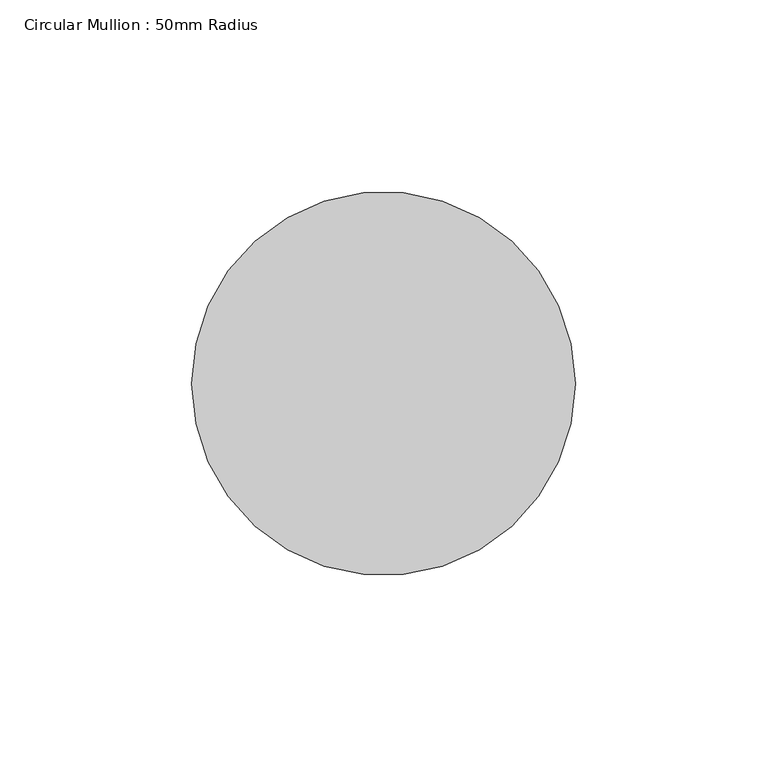
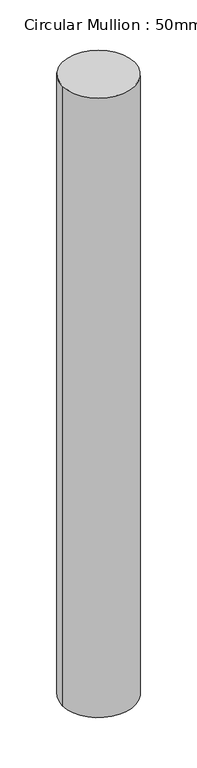
"""IFC4 building model written with IfcOpenShell, lengths in millimetres: member geometry, Circular Mullion : 50mm Radius."""

from ifc_helpers import new_model, si_unit, point, frame, origin, origin_2d, place, context, project, spatial, circle_curve, trimmed, segment, composite_curve, outline, extrude, source, transform, mapped, element, save


def circular_mullion_50mm_radius_d6f7776c(model_context):
    return source(origin(), model_context, "Body", "SweptSolid", [
        extrude(outline(composite_curve([segment(trimmed(circle_curve(origin_2d(), 50.0), [point((50.0, 0.0))], [point((-50.0, 0.0))], False, "CARTESIAN"), True, "CONTINUOUS"), segment(trimmed(circle_curve(origin_2d(), 50.0), [point((-50.0, 0.0))], [point((50.0, 0.0))], False, "CARTESIAN"), True, "CONTINUOUS")], self_intersect=False)), frame((0.0, 0.0, -908.470151), z_axis=(0.0, 0.0, 1.0), x_axis=(1.0, 0.0, 0.0)), (0.0, 0.0, 1.0), 908.470151),
    ])


if __name__ == "__main__":
    model = new_model("IFC4")
    model_context = context("Model", 3, world=origin())
    ifc_project = project(units=[si_unit("LENGTHUNIT", "METRE", prefix="MILLI")], contexts=[model_context])
    site = spatial("IfcSite", under=ifc_project)
    building = spatial("IfcBuilding", under=site)
    placement = place(None, origin())
    circular_mullion_50mm_radius_shape = circular_mullion_50mm_radius_d6f7776c(model_context)
    element("IfcMember", 1, ObjectType="Circular Mullion : 50mm Radius", at=placement, inside=building, context=model_context, shape_type="MappedRepresentation", body=[
        mapped(circular_mullion_50mm_radius_shape, transform((0.0, 0.0, 0.0), x_axis=(1.0, 0.0, 0.0), y_axis=(0.0, 1.0, 0.0), z_axis=(0.0, 0.0, 1.0))),
    ])
    save(model, "model.ifc")

# Revit data of these elements
# Type "Circular Mullion : 50mm Radius"
#   built-in parameter 1007350 = 0.164042 (stored number, unit not read)
# Element 1 (IfcMember, "Circular Mullion : 50mm Radius")
#   Materials on its faces: "Aluminium"
# Materials
#   "Aluminium": class "Metal", colour RGB 247 247 247, transparency 0, Description = "Aluminium 6061", Cost = 0
